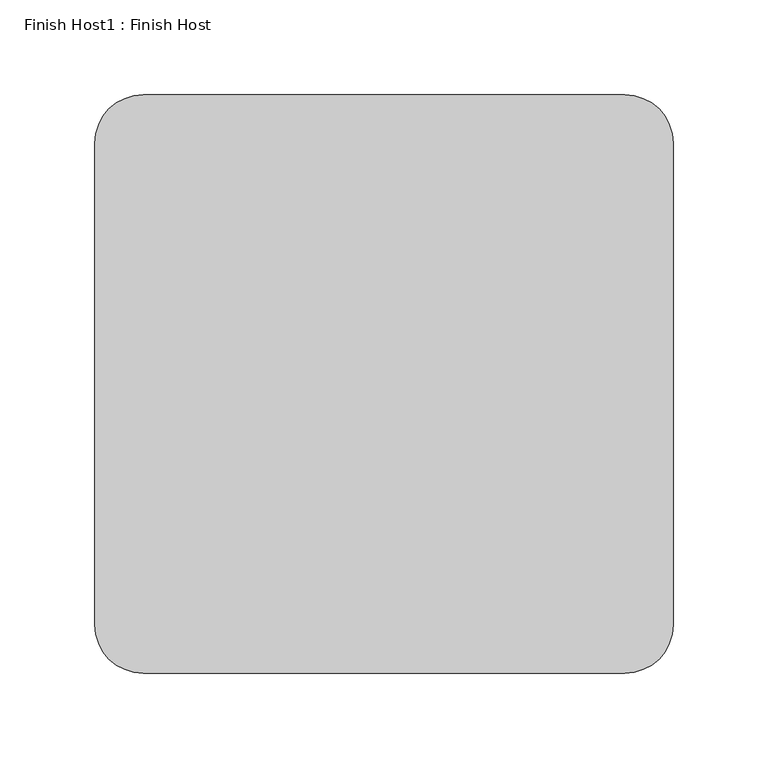
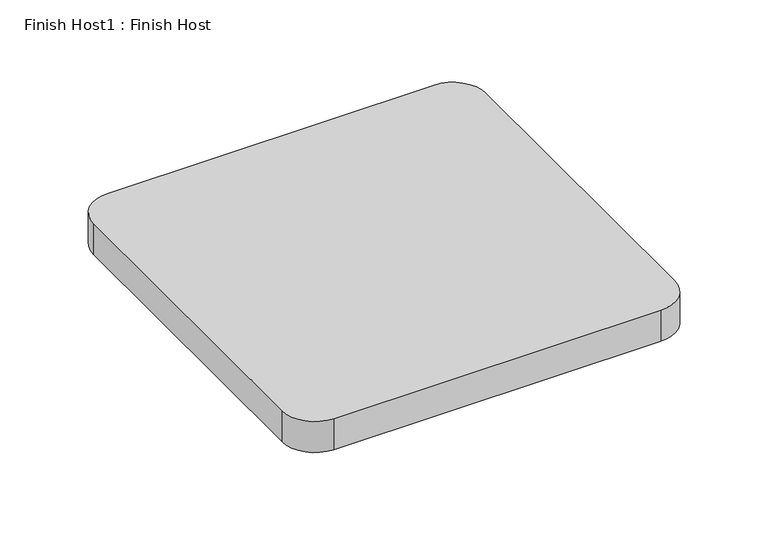
"""IFC4 building model written with IfcOpenShell, lengths in millimetres: proxy geometry, Finish Host1 : Finish Host."""

from ifc_helpers import new_model, si_unit, point, frame_2d, origin, origin_with_axes, place, context, project, spatial, polyline, circle_curve, trimmed, segment, composite_curve, outline, extrude, source, transform, mapped, element, save


def finish_host1_finish_host_d3433be2(model_context):
    return source(origin(), model_context, "Body", "SweptSolid", [
        extrude(outline(composite_curve([segment(polyline([(-797.1842816, 4229.4760864), (-797.1842816, 4483.4760864)]), True, "CONTINUOUS"), segment(trimmed(circle_curve(frame_2d((-771.7842816, 4483.4760864)), 25.4), [point((-797.1842816, 4483.4760864))], [point((-771.7842816, 4508.8760864))], False, "CARTESIAN"), True, "CONTINUOUS"), segment(polyline([(-771.7842816, 4508.8760864), (-517.7842816, 4508.8760864)]), True, "CONTINUOUS"), segment(trimmed(circle_curve(frame_2d((-517.7842816, 4483.4760864)), 25.4), [point((-517.7842816, 4508.8760864))], [point((-492.3842816, 4483.4760864))], False, "CARTESIAN"), True, "CONTINUOUS"), segment(polyline([(-492.3842816, 4483.4760864), (-492.3842816, 4229.4760864)]), True, "CONTINUOUS"), segment(trimmed(circle_curve(frame_2d((-517.7842816, 4229.4760864)), 25.4), [point((-492.3842816, 4229.4760864))], [point((-517.7842816, 4204.0760864))], False, "CARTESIAN"), True, "CONTINUOUS"), segment(polyline([(-517.7842816, 4204.0760864), (-771.7842816, 4204.0760864)]), True, "CONTINUOUS"), segment(trimmed(circle_curve(frame_2d((-771.7842816, 4229.4760864)), 25.4), [point((-771.7842816, 4204.0760864))], [point((-797.1842816, 4229.4760864))], False, "CARTESIAN"), True, "CONTINUOUS")], self_intersect=False)), origin_with_axes(), (0.0, 0.0, 1.0), 25.4),
    ])


if __name__ == "__main__":
    model = new_model("IFC4")
    model_context = context("Model", 3, world=origin())
    ifc_project = project(units=[si_unit("LENGTHUNIT", "METRE", prefix="MILLI")], contexts=[model_context])
    site = spatial("IfcSite", under=ifc_project)
    building = spatial("IfcBuilding", under=site)
    placement = place(None, origin())
    finish_host1_finish_host_shape = finish_host1_finish_host_d3433be2(model_context)
    element("IfcBuildingElementProxy", 1, Name="Finish Host1 : Finish Host", ObjectType="Finish Host1 : Finish Host", at=placement, inside=building, context=model_context, shape_type="MappedRepresentation", body=[
        mapped(finish_host1_finish_host_shape, transform((0.0, 0.0, 0.0), x_axis=(1.0, 0.0, 0.0), y_axis=(0.0, 1.0, 0.0), z_axis=(0.0, 0.0, 1.0))),
    ])
    save(model, "model.ifc")

# Revit data of these elements
# Type "Finish Host1 : Finish Host"
#   Panel Material = Fabric - Teknion - S135 - Synaptic - Contact
# Element 1 (IfcBuildingElementProxy, "Finish Host1 : Finish Host")
#   Materials on its faces: "Fabric - Teknion - S135 - Synaptic - Contact"
# Materials
#   "Fabric - Teknion - S135 - Synaptic - Contact": class "Fabric", colour RGB 53 52 51, transparency 0, Model = "S135", Manufacturer = "Teknion Studio", URL = "http://www.teknionstudio.com/", Description = "Contact Synaptic", Cost = 0
